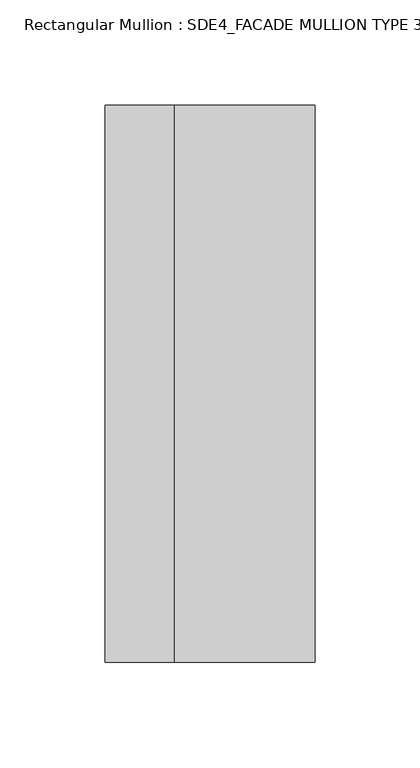
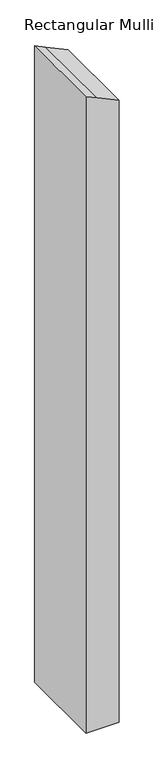
"""IFC4 building model written with IfcOpenShell, lengths in millimetres: member geometry, Rectangular Mullion : SDE4_FACADE MULLION TYPE 3."""

import ifcopenshell
import ifcopenshell.guid

model = None  # the IFC model being written
_history = None  # IfcOwnerHistory: only IFC2X3 demands one
_inside = {}  # id of a spatial element -> (the spatial element, [elements in it])
_under = {}  # id of a project, library or spatial element -> (it, [spatial elements below it])
_declared = {}  # id of a project -> (the project, [libraries it declares])
_typed = {}  # id of a type object -> (the type object, [elements of that type])
_made_of = {}  # id of a material, layer set ... -> (it, [elements and type objects made of it])


def new_model(schema):
    """Start an empty IFC model of exactly this schema.

    Asked for "IFC4X3", IfcOpenShell would pick the latest addendum, in which some entities
    have other attributes; the version numbers below select the first issue.
    IFC2X3 requires an IfcOwnerHistory on every rooted entity: one is made here for all.
    """
    global model, _history
    if schema == "IFC4X3":
        model = ifcopenshell.file(schema_version=(4, 3, 0, 0))
    else:
        model = ifcopenshell.file(schema=schema)
    _inside.clear()
    _under.clear()
    _declared.clear()
    _typed.clear()
    _made_of.clear()
    _history = None
    if model.schema == "IFC2X3":
        org = make("IfcOrganization", Name="unknown")
        user = make(
            "IfcPersonAndOrganization",
            ThePerson=make("IfcPerson", FamilyName="unknown"),
            TheOrganization=org,
        )
        app = make(
            "IfcApplication",
            ApplicationDeveloper=org,
            Version="unknown",
            ApplicationFullName="unknown",
            ApplicationIdentifier="unknown",
        )
        _history = make(
            "IfcOwnerHistory",
            OwningUser=user,
            OwningApplication=app,
            ChangeAction="ADDED",
            CreationDate=0,
        )
    return model


def make(cls, **values):
    """One entity of the class cls with the attributes given. An attribute that is None is left unset."""
    return model.create_entity(
        cls, **{name: value for name, value in values.items() if value is not None}
    )


def rooted(cls, **values):
    """An entity with a GlobalId (a new one), such as an element, a storey or a relation."""
    return make(cls, GlobalId=ifcopenshell.guid.new(), OwnerHistory=_history, **values)


def si_unit(unit_type, name, prefix=None):
    """IfcSIUnit, for example si_unit("LENGTHUNIT", "METRE", prefix="MILLI")."""
    return make("IfcSIUnit", UnitType=unit_type, Prefix=prefix, Name=name)


def assignment(units):
    """IfcUnitAssignment: the units of a project."""
    return None if units is None else make("IfcUnitAssignment", Units=units)


def point(xyz):
    """IfcCartesianPoint."""
    return None if xyz is None else make("IfcCartesianPoint", Coordinates=xyz)


def direction(xyz):
    """IfcDirection."""
    return None if xyz is None else make("IfcDirection", DirectionRatios=xyz)


def frame(location, z_axis=None, x_axis=None):
    """IfcAxis2Placement3D, a coordinate frame: its origin and axes. An axis left out is left unset."""
    return make(
        "IfcAxis2Placement3D",
        Location=point(location),
        Axis=direction(z_axis),
        RefDirection=direction(x_axis),
    )


def origin():
    """The frame at (0, 0, 0) with its axes left unset."""
    return frame((0.0, 0.0, 0.0))


def place(relative_to, where):
    """IfcLocalPlacement: puts the frame where relative to a parent placement (None: the world)."""
    return make(
        "IfcLocalPlacement", PlacementRelTo=relative_to, RelativePlacement=where
    )


def context(
    kind, dimensions, precision=None, world=None, true_north=None, identifier=None
):
    """IfcGeometricRepresentationContext, for example the 3D "Model" context."""
    return make(
        "IfcGeometricRepresentationContext",
        ContextIdentifier=identifier,
        ContextType=kind,
        CoordinateSpaceDimension=dimensions,
        Precision=precision,
        WorldCoordinateSystem=world,
        TrueNorth=true_north,
    )


def project(units=None, contexts=None):
    """IfcProject with its units and contexts."""
    return rooted(
        "IfcProject",
        Name="project",
        RepresentationContexts=contexts,
        UnitsInContext=assignment(units),
    )


def spatial(cls, under=None, at=None, **own):
    """A site, building, storey or space (cls), placed at a placement, below another one or the project."""
    s = rooted(cls, ObjectPlacement=at, **own)
    if under is not None:
        _under.setdefault(under.id(), (under, []))[1].append(s)
    return s


def polyline(points):
    """IfcPolyline through the points."""
    return make("IfcPolyline", Points=[point(p) for p in points])


def outline(outer, holes=None, kind="AREA"):
    """IfcArbitraryClosedProfileDef: a profile drawn as a closed curve; with holes, ...WithVoids."""
    if holes is None:
        return make("IfcArbitraryClosedProfileDef", ProfileType=kind, OuterCurve=outer)
    return make(
        "IfcArbitraryProfileDefWithVoids",
        ProfileType=kind,
        OuterCurve=outer,
        InnerCurves=holes,
    )


def extrude(swept, where, along, depth):
    """IfcExtrudedAreaSolid: the profile swept, set in the frame where, extruded along a direction by depth."""
    return make(
        "IfcExtrudedAreaSolid",
        SweptArea=swept,
        Position=where,
        ExtrudedDirection=direction(along),
        Depth=depth,
    )


def shape(context_of_items, identifier, shape_type, items):
    """IfcShapeRepresentation: the items that make up one representation, for example the "Body"."""
    return make(
        "IfcShapeRepresentation",
        ContextOfItems=context_of_items,
        RepresentationIdentifier=identifier,
        RepresentationType=shape_type,
        Items=items,
    )


def source(mapping_origin, context_of_items, identifier, shape_type, items):
    """IfcRepresentationMap: a shape defined once, which mapped items show again and again."""
    return make(
        "IfcRepresentationMap",
        MappingOrigin=mapping_origin,
        MappedRepresentation=shape(context_of_items, identifier, shape_type, items),
    )


def transform(
    local_origin,
    x_axis=None,
    y_axis=None,
    z_axis=None,
    scale=None,
    scale2=None,
    scale3=None,
    uniform=True,
):
    """IfcCartesianTransformationOperator3D, or its non-uniform kind. x_axis, y_axis, z_axis: its Axis1, 2, 3."""
    if uniform:
        return make(
            "IfcCartesianTransformationOperator3D",
            Axis1=direction(x_axis),
            Axis2=direction(y_axis),
            LocalOrigin=point(local_origin),
            Scale=scale,
            Axis3=direction(z_axis),
        )
    return make(
        "IfcCartesianTransformationOperator3DnonUniform",
        Axis1=direction(x_axis),
        Axis2=direction(y_axis),
        LocalOrigin=point(local_origin),
        Scale=scale,
        Axis3=direction(z_axis),
        Scale2=scale2,
        Scale3=scale3,
    )


def mapped(mapping_source, mapping_target):
    """IfcMappedItem: shows the shape of a source again, moved by a transform."""
    return make(
        "IfcMappedItem", MappingSource=mapping_source, MappingTarget=mapping_target
    )


def made_of(thing, what):
    """Note that an element or type object is made of a material, layer set ...; save() writes the relation."""
    if what is not None:
        _made_of.setdefault(what.id(), (what, []))[1].append(thing)
    return thing


def element(
    cls,
    number,
    at=None,
    inside=None,
    cuts=None,
    type_object=None,
    material=None,
    context=None,
    identifier="Body",
    shape_type=None,
    held_by="IfcProductDefinitionShape",
    body=None,
    shapes=None,
    **own,
):
    """One element of the class cls, such as IfcWall. Its Tag is "e" and its number.

    at: its placement. inside: the storey or other place that contains it. cuts: it is an
    opening in that element (IfcRelVoidsElement). A single representation is given by context,
    identifier, shape_type and body (its items); several are given by shapes. held_by: the class
    of the entity that holds the representations. save() writes the other relations.
    """
    e = rooted(cls, Tag="e%d" % number, ObjectPlacement=at, **own)
    if body is not None:
        shapes = [shape(context, identifier, shape_type, body)]
    if shapes is not None:
        e.Representation = make(held_by, Representations=shapes)
    if inside is not None:
        _inside.setdefault(inside.id(), (inside, []))[1].append(e)
    if cuts is not None:
        rooted(
            "IfcRelVoidsElement", RelatingBuildingElement=cuts, RelatedOpeningElement=e
        )
    if type_object is not None:
        _typed.setdefault(type_object.id(), (type_object, []))[1].append(e)
    return made_of(e, material)


def aggregate(whole, parts):
    """IfcRelAggregates: a whole, such as a stair, and the parts it consists of."""
    return rooted("IfcRelAggregates", RelatingObject=whole, RelatedObjects=parts)


def save(model, path):
    """Write the relations noted so far, then the file.

    IfcRelAggregates (storeys below a building ...), IfcRelContainedInSpatialStructure (elements
    in a storey), IfcRelDefinesByType, IfcRelAssociatesMaterial and IfcRelDeclares: one each for
    every whole, place, type object, material and project.
    """
    for whole, parts in _under.values():
        aggregate(whole, parts)
    for where, things in _inside.values():
        rooted(
            "IfcRelContainedInSpatialStructure",
            RelatedElements=things,
            RelatingStructure=where,
        )
    for kind, things in _typed.values():
        rooted("IfcRelDefinesByType", RelatedObjects=things, RelatingType=kind)
    for what, things in _made_of.values():
        rooted("IfcRelAssociatesMaterial", RelatedObjects=things, RelatingMaterial=what)
    for by, libraries in _declared.values():
        rooted("IfcRelDeclares", RelatingContext=by, RelatedDefinitions=libraries)
    model.write(path)


def rectangular_mullion_sde4_facade_mullion_type_3_1ed854a7(model_context):
    return source(origin(), model_context, "Body", "SweptSolid", [
        extrude(outline(polyline([(-67.4504667, 50.0), (-36.2523183, -16.9047158), (-20.8197502, -50.0), (-2034.9759037, -50.0), (-2034.9759037, 50.0), (-67.4504667, 50.0)])), frame((0.0, -132.5, 0.0), z_axis=(0.0, 1.0, 0.0), x_axis=(0.0, 0.0, 1.0)), (0.0, 0.0, 1.0), 265.0),
    ])


if __name__ == "__main__":
    model = new_model("IFC4")
    model_context = context("Model", 3, world=origin())
    ifc_project = project(units=[si_unit("LENGTHUNIT", "METRE", prefix="MILLI")], contexts=[model_context])
    site = spatial("IfcSite", under=ifc_project)
    building = spatial("IfcBuilding", under=site)
    placement = place(None, origin())
    rectangular_mullion_sde4_facade_mullion_type_3_shape = rectangular_mullion_sde4_facade_mullion_type_3_1ed854a7(model_context)
    element("IfcMember", 1, ObjectType="Rectangular Mullion : SDE4_FACADE MULLION TYPE 3", at=placement, inside=building, context=model_context, shape_type="MappedRepresentation", body=[
        mapped(rectangular_mullion_sde4_facade_mullion_type_3_shape, transform((0.0, 0.0, 0.0), x_axis=(1.0, 0.0, 0.0), y_axis=(0.0, 1.0, 0.0), z_axis=(0.0, 0.0, 1.0))),
    ])
    save(model, "model.ifc")

# Revit data of these elements
# Type "Rectangular Mullion : SDE4_FACADE MULLION TYPE 3"
#   built-in parameter 1007322 = 0.869423 (stored number, unit not read)
#   built-in parameter 1007321 = 0.164042 (stored number, unit not read)
#   built-in parameter 1007320 = 0.164042 (stored number, unit not read)
